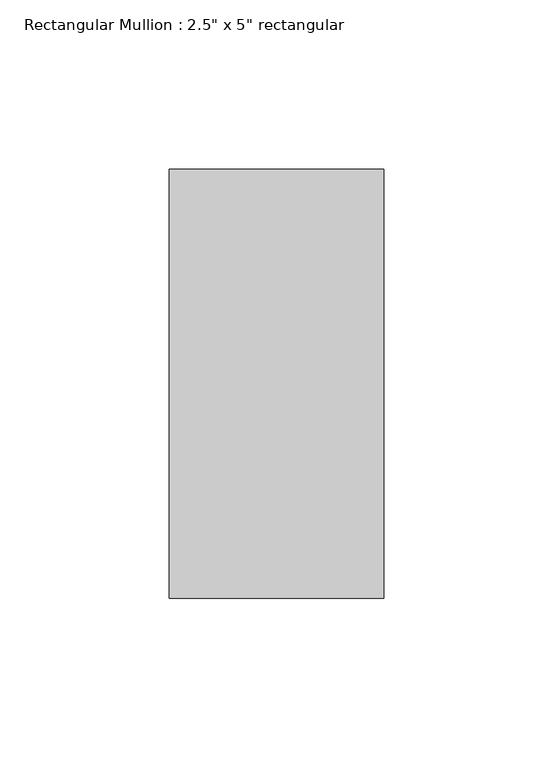
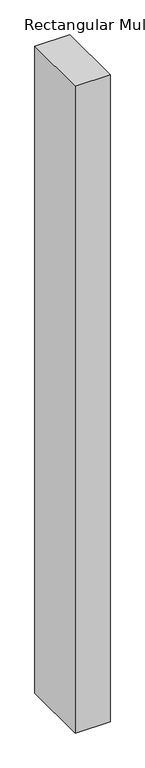
"""IFC4 building model written with IfcOpenShell, lengths in millimetres: member geometry."""

from ifc_helpers import new_model, si_unit, frame, origin, place, context, project, spatial, polyline, outline, extrude, source, transform, mapped, element, save


def member_59c53a79(model_context):
    return source(origin(), model_context, "Body", "SweptSolid", [
        extrude(outline(polyline([(0.0, 63.5), (0.0, -63.5), (-63.5, -63.5), (-63.5, 63.5), (0.0, 63.5)])), frame((0.0, 0.0, -1245.39375), z_axis=(0.0, 0.0, 1.0), x_axis=(1.0, 0.0, 0.0)), (0.0, 0.0, 1.0), 1245.39375),
    ])


if __name__ == "__main__":
    model = new_model("IFC4")
    model_context = context("Model", 3, world=origin())
    ifc_project = project(units=[si_unit("LENGTHUNIT", "METRE", prefix="MILLI")], contexts=[model_context])
    site = spatial("IfcSite", under=ifc_project)
    building = spatial("IfcBuilding", under=site)
    placement = place(None, origin())
    member_shape = member_59c53a79(model_context)
    element("IfcMember", 1, ObjectType="Rectangular Mullion : 2.5\" x 5\" rectangular", at=placement, inside=building, context=model_context, shape_type="MappedRepresentation", body=[
        mapped(member_shape, transform((0.0, 0.0, 0.0), x_axis=(1.0, 0.0, 0.0), y_axis=(0.0, 1.0, 0.0), z_axis=(0.0, 0.0, 1.0))),
    ])
    save(model, "model.ifc")

# Revit data of these elements
# Type "Rectangular Mullion : 2.5\" x 5\" rectangular"
#   built-in parameter 1007304 = 0.416667 (stored number, unit not read)
#   built-in parameter 1007301 = 0.104167 (stored number, unit not read)
#   built-in parameter 1007300 = 0.104167 (stored number, unit not read)
# Element 1 (IfcMember, "Rectangular Mullion : 2.5\" x 5\" rectangular")
#   Materials on its faces: "Metal - Aluminum"
# Materials
#   "Metal - Aluminum": class "Metal", colour RGB 140 140 140, transparency 0
